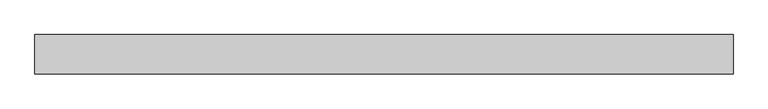
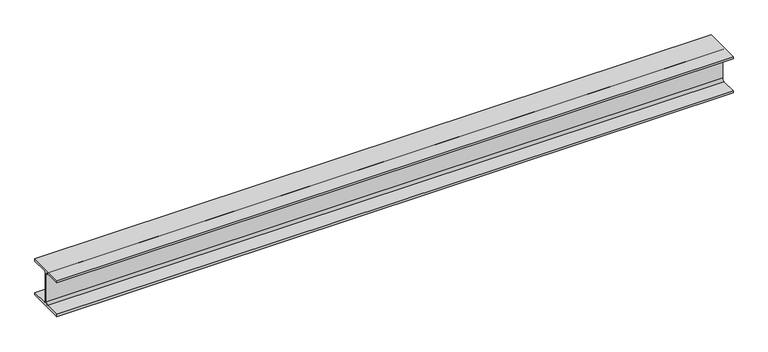
"""IFC4 building model written with IfcOpenShell, lengths in millimetres: beam geometry, 0912_Steel Framing_H-KSD3502 : H_SB_ASB_H-200x200x8x12."""

import ifcopenshell
import ifcopenshell.guid

model = None  # the IFC model being written
_history = None  # IfcOwnerHistory: only IFC2X3 demands one
_inside = {}  # id of a spatial element -> (the spatial element, [elements in it])
_under = {}  # id of a project, library or spatial element -> (it, [spatial elements below it])
_declared = {}  # id of a project -> (the project, [libraries it declares])
_typed = {}  # id of a type object -> (the type object, [elements of that type])
_made_of = {}  # id of a material, layer set ... -> (it, [elements and type objects made of it])


def new_model(schema):
    """Start an empty IFC model of exactly this schema.

    Asked for "IFC4X3", IfcOpenShell would pick the latest addendum, in which some entities
    have other attributes; the version numbers below select the first issue.
    IFC2X3 requires an IfcOwnerHistory on every rooted entity: one is made here for all.
    """
    global model, _history
    if schema == "IFC4X3":
        model = ifcopenshell.file(schema_version=(4, 3, 0, 0))
    else:
        model = ifcopenshell.file(schema=schema)
    _inside.clear()
    _under.clear()
    _declared.clear()
    _typed.clear()
    _made_of.clear()
    _history = None
    if model.schema == "IFC2X3":
        org = make("IfcOrganization", Name="unknown")
        user = make(
            "IfcPersonAndOrganization",
            ThePerson=make("IfcPerson", FamilyName="unknown"),
            TheOrganization=org,
        )
        app = make(
            "IfcApplication",
            ApplicationDeveloper=org,
            Version="unknown",
            ApplicationFullName="unknown",
            ApplicationIdentifier="unknown",
        )
        _history = make(
            "IfcOwnerHistory",
            OwningUser=user,
            OwningApplication=app,
            ChangeAction="ADDED",
            CreationDate=0,
        )
    return model


def make(cls, **values):
    """One entity of the class cls with the attributes given. An attribute that is None is left unset."""
    return model.create_entity(
        cls, **{name: value for name, value in values.items() if value is not None}
    )


def rooted(cls, **values):
    """An entity with a GlobalId (a new one), such as an element, a storey or a relation."""
    return make(cls, GlobalId=ifcopenshell.guid.new(), OwnerHistory=_history, **values)


def si_unit(unit_type, name, prefix=None):
    """IfcSIUnit, for example si_unit("LENGTHUNIT", "METRE", prefix="MILLI")."""
    return make("IfcSIUnit", UnitType=unit_type, Prefix=prefix, Name=name)


def assignment(units):
    """IfcUnitAssignment: the units of a project."""
    return None if units is None else make("IfcUnitAssignment", Units=units)


def point(xyz):
    """IfcCartesianPoint."""
    return None if xyz is None else make("IfcCartesianPoint", Coordinates=xyz)


def direction(xyz):
    """IfcDirection."""
    return None if xyz is None else make("IfcDirection", DirectionRatios=xyz)


def frame(location, z_axis=None, x_axis=None):
    """IfcAxis2Placement3D, a coordinate frame: its origin and axes. An axis left out is left unset."""
    return make(
        "IfcAxis2Placement3D",
        Location=point(location),
        Axis=direction(z_axis),
        RefDirection=direction(x_axis),
    )


def frame_2d(location, x_axis=None):
    """IfcAxis2Placement2D, a coordinate frame in the plane: its origin and x axis."""
    return make(
        "IfcAxis2Placement2D", Location=point(location), RefDirection=direction(x_axis)
    )


def origin():
    """The frame at (0, 0, 0) with its axes left unset."""
    return frame((0.0, 0.0, 0.0))


def place(relative_to, where):
    """IfcLocalPlacement: puts the frame where relative to a parent placement (None: the world)."""
    return make(
        "IfcLocalPlacement", PlacementRelTo=relative_to, RelativePlacement=where
    )


def context(
    kind, dimensions, precision=None, world=None, true_north=None, identifier=None
):
    """IfcGeometricRepresentationContext, for example the 3D "Model" context."""
    return make(
        "IfcGeometricRepresentationContext",
        ContextIdentifier=identifier,
        ContextType=kind,
        CoordinateSpaceDimension=dimensions,
        Precision=precision,
        WorldCoordinateSystem=world,
        TrueNorth=true_north,
    )


def project(units=None, contexts=None):
    """IfcProject with its units and contexts."""
    return rooted(
        "IfcProject",
        Name="project",
        RepresentationContexts=contexts,
        UnitsInContext=assignment(units),
    )


def spatial(cls, under=None, at=None, **own):
    """A site, building, storey or space (cls), placed at a placement, below another one or the project."""
    s = rooted(cls, ObjectPlacement=at, **own)
    if under is not None:
        _under.setdefault(under.id(), (under, []))[1].append(s)
    return s


def polyline(points):
    """IfcPolyline through the points."""
    return make("IfcPolyline", Points=[point(p) for p in points])


def circle_curve(where, radius):
    """IfcCircle in the frame where."""
    return make("IfcCircle", Position=where, Radius=radius)


def trimmed(basis, trim1, trim2, sense, master):
    """IfcTrimmedCurve: the piece of a basis curve between two trims."""
    return make(
        "IfcTrimmedCurve",
        BasisCurve=basis,
        Trim1=trim1,
        Trim2=trim2,
        SenseAgreement=sense,
        MasterRepresentation=master,
    )


def segment(curve, same_sense, transition):
    """IfcCompositeCurveSegment."""
    return make(
        "IfcCompositeCurveSegment",
        Transition=transition,
        SameSense=same_sense,
        ParentCurve=curve,
    )


def composite_curve(segments, self_intersect=None):
    """IfcCompositeCurve: segments joined end to end."""
    return make("IfcCompositeCurve", Segments=segments, SelfIntersect=self_intersect)


def outline(outer, holes=None, kind="AREA"):
    """IfcArbitraryClosedProfileDef: a profile drawn as a closed curve; with holes, ...WithVoids."""
    if holes is None:
        return make("IfcArbitraryClosedProfileDef", ProfileType=kind, OuterCurve=outer)
    return make(
        "IfcArbitraryProfileDefWithVoids",
        ProfileType=kind,
        OuterCurve=outer,
        InnerCurves=holes,
    )


def extrude(swept, where, along, depth):
    """IfcExtrudedAreaSolid: the profile swept, set in the frame where, extruded along a direction by depth."""
    return make(
        "IfcExtrudedAreaSolid",
        SweptArea=swept,
        Position=where,
        ExtrudedDirection=direction(along),
        Depth=depth,
    )


def shape(context_of_items, identifier, shape_type, items):
    """IfcShapeRepresentation: the items that make up one representation, for example the "Body"."""
    return make(
        "IfcShapeRepresentation",
        ContextOfItems=context_of_items,
        RepresentationIdentifier=identifier,
        RepresentationType=shape_type,
        Items=items,
    )


def source(mapping_origin, context_of_items, identifier, shape_type, items):
    """IfcRepresentationMap: a shape defined once, which mapped items show again and again."""
    return make(
        "IfcRepresentationMap",
        MappingOrigin=mapping_origin,
        MappedRepresentation=shape(context_of_items, identifier, shape_type, items),
    )


def transform(
    local_origin,
    x_axis=None,
    y_axis=None,
    z_axis=None,
    scale=None,
    scale2=None,
    scale3=None,
    uniform=True,
):
    """IfcCartesianTransformationOperator3D, or its non-uniform kind. x_axis, y_axis, z_axis: its Axis1, 2, 3."""
    if uniform:
        return make(
            "IfcCartesianTransformationOperator3D",
            Axis1=direction(x_axis),
            Axis2=direction(y_axis),
            LocalOrigin=point(local_origin),
            Scale=scale,
            Axis3=direction(z_axis),
        )
    return make(
        "IfcCartesianTransformationOperator3DnonUniform",
        Axis1=direction(x_axis),
        Axis2=direction(y_axis),
        LocalOrigin=point(local_origin),
        Scale=scale,
        Axis3=direction(z_axis),
        Scale2=scale2,
        Scale3=scale3,
    )


def mapped(mapping_source, mapping_target):
    """IfcMappedItem: shows the shape of a source again, moved by a transform."""
    return make(
        "IfcMappedItem", MappingSource=mapping_source, MappingTarget=mapping_target
    )


def made_of(thing, what):
    """Note that an element or type object is made of a material, layer set ...; save() writes the relation."""
    if what is not None:
        _made_of.setdefault(what.id(), (what, []))[1].append(thing)
    return thing


def element(
    cls,
    number,
    at=None,
    inside=None,
    cuts=None,
    type_object=None,
    material=None,
    context=None,
    identifier="Body",
    shape_type=None,
    held_by="IfcProductDefinitionShape",
    body=None,
    shapes=None,
    **own,
):
    """One element of the class cls, such as IfcWall. Its Tag is "e" and its number.

    at: its placement. inside: the storey or other place that contains it. cuts: it is an
    opening in that element (IfcRelVoidsElement). A single representation is given by context,
    identifier, shape_type and body (its items); several are given by shapes. held_by: the class
    of the entity that holds the representations. save() writes the other relations.
    """
    e = rooted(cls, Tag="e%d" % number, ObjectPlacement=at, **own)
    if body is not None:
        shapes = [shape(context, identifier, shape_type, body)]
    if shapes is not None:
        e.Representation = make(held_by, Representations=shapes)
    if inside is not None:
        _inside.setdefault(inside.id(), (inside, []))[1].append(e)
    if cuts is not None:
        rooted(
            "IfcRelVoidsElement", RelatingBuildingElement=cuts, RelatedOpeningElement=e
        )
    if type_object is not None:
        _typed.setdefault(type_object.id(), (type_object, []))[1].append(e)
    return made_of(e, material)


def aggregate(whole, parts):
    """IfcRelAggregates: a whole, such as a stair, and the parts it consists of."""
    return rooted("IfcRelAggregates", RelatingObject=whole, RelatedObjects=parts)


def save(model, path):
    """Write the relations noted so far, then the file.

    IfcRelAggregates (storeys below a building ...), IfcRelContainedInSpatialStructure (elements
    in a storey), IfcRelDefinesByType, IfcRelAssociatesMaterial and IfcRelDeclares: one each for
    every whole, place, type object, material and project.
    """
    for whole, parts in _under.values():
        aggregate(whole, parts)
    for where, things in _inside.values():
        rooted(
            "IfcRelContainedInSpatialStructure",
            RelatedElements=things,
            RelatingStructure=where,
        )
    for kind, things in _typed.values():
        rooted("IfcRelDefinesByType", RelatedObjects=things, RelatingType=kind)
    for what, things in _made_of.values():
        rooted("IfcRelAssociatesMaterial", RelatedObjects=things, RelatingMaterial=what)
    for by, libraries in _declared.values():
        rooted("IfcRelDeclares", RelatingContext=by, RelatedDefinitions=libraries)
    model.write(path)


def beam_9e25a490(model_context):
    return source(origin(), model_context, "Body", "SweptSolid", [
        extrude(outline(composite_curve([segment(polyline([(100.0, -88.0), (100.0, -100.0), (-100.0, -100.0), (-100.0, -88.0), (-17.0, -88.0)]), True, "CONTINUOUS"), segment(trimmed(circle_curve(frame_2d((-17.0, -75.0)), 13.0), [point((-17.0, -88.0))], [point((-4.0, -75.0))], True, "CARTESIAN"), True, "CONTINUOUS"), segment(polyline([(-4.0, -75.0), (-4.0, 75.0)]), True, "CONTINUOUS"), segment(trimmed(circle_curve(frame_2d((-17.0, 75.0)), 13.0), [point((-4.0, 75.0))], [point((-17.0, 88.0))], True, "CARTESIAN"), True, "CONTINUOUS"), segment(polyline([(-17.0, 88.0), (-100.0, 88.0), (-100.0, 100.0), (100.0, 100.0), (100.0, 88.0), (17.0, 88.0)]), True, "CONTINUOUS"), segment(trimmed(circle_curve(frame_2d((17.0, 75.0)), 13.0), [point((17.0, 88.0))], [point((4.0, 75.0))], True, "CARTESIAN"), True, "CONTINUOUS"), segment(polyline([(4.0, 75.0), (4.0, -75.0)]), True, "CONTINUOUS"), segment(trimmed(circle_curve(frame_2d((17.0, -75.0)), 13.0), [point((4.0, -75.0))], [point((17.0, -88.0))], True, "CARTESIAN"), True, "CONTINUOUS"), segment(polyline([(17.0, -88.0), (100.0, -88.0)]), True, "CONTINUOUS")], self_intersect=False)), frame((-1734.3504002, 0.0, 0.0), z_axis=(1.0, 0.0, 0.0), x_axis=(0.0, 1.0, 0.0)), (0.0, 0.0, 1.0), 3554.555596),
    ])


if __name__ == "__main__":
    model = new_model("IFC4")
    model_context = context("Model", 3, world=origin())
    ifc_project = project(units=[si_unit("LENGTHUNIT", "METRE", prefix="MILLI")], contexts=[model_context])
    site = spatial("IfcSite", under=ifc_project)
    building = spatial("IfcBuilding", under=site)
    placement = place(None, origin())
    beam_shape = beam_9e25a490(model_context)
    element("IfcBeam", 1, ObjectType="0912_Steel Framing_H-KSD3502 : H_SB_ASB_H-200x200x8x12", at=placement, inside=building, context=model_context, shape_type="MappedRepresentation", body=[
        mapped(beam_shape, transform((0.0, 0.0, 0.0), x_axis=(1.0, 0.0, 0.0), y_axis=(0.0, 1.0, 0.0), z_axis=(0.0, 0.0, 1.0))),
    ])
    save(model, "model.ifc")

# Revit data of these elements
# Type "0912_Steel Framing_H-KSD3502 : H_SB_ASB_H-200x200x8x12"
#   H_WM Code_1 = "S01AA002-00001 | Main Steel Structure Fabrication Work | Shelter/Building | Medium Steel - Standard (90KG/M>Weight≥30KG/M) | Material: (   )"
#   H_WM Code_2 = "S03AA028-00001 | Main Steel Structure Erection Work | Shelter/Building | Medium Steel (90KG/M>Weight≥30KG/M) | Material: (   )"
#   H_WM Code_3 = "S01AA010-00001 | Main Steel Structure Fabrication Work | Shelter/Building | Steel Painting/Coating | for Non-Fireproofed Steel Surface, Surface Preparation, Primer, Second & Final Coat | Material: (   )"
#   H_Q'ty Cal Type Tag = "SB-Q2"
#   Width = 20.0 cm
#   Web Thickness = 0.8 cm
#   Web Fillet = 1.3 cm
#   Warping Constant = 141000.0 cm⁶
#   W = 0
#   Torsional Moment of Inertia = 26.2485 cm⁴
#   Section Area = 63.53 cm²
#   Plastic Modulus weak axis = 244.0 cm³
#   Plastic Modulus strong axis = 525.0 cm³
#   Perimeter = 1.16 m²/m
#   Nominal Weight = 49.90 kgf/m
#   Moment of Inertia weak axis = 1600.00 cm⁴
#   Moment of Inertia strong axis = 4720.00 cm⁴
#   Height = 20.0 cm
#   Flange Thickness = 1.2 cm
#   Elastic Modulus weak axis = 160.0 cm³
#   Elastic Modulus strong axis = 472.0 cm³
#   Centroid Vertical = 10.0 cm
#   Centroid Horizontal = 10.0 cm
#   Ix = 47200000
#   Length [instance default] = 1.5240 m
#   Zx = 525000
#   b = 0.2000 m
#   h = 0.2000 m
#   r = 0.0130 m
#   s = 0.0080 m
#   t = 0.0120 m
#   A = 0.006353 m²
#   Structural Material [instance default] = Steel, 45-345
#   Assembly Code = ""
# Element 1 (IfcBeam, "0912_Steel Framing_H-KSD3502 : H_SB_ASB_H-200x200x8x12")
#   Structural Material = none
# Materials
#   "Steel, 45-345": class "Metal", colour RGB 189 187 185, transparency 0, Description = "Steel 345 MPa", Cost = 0
